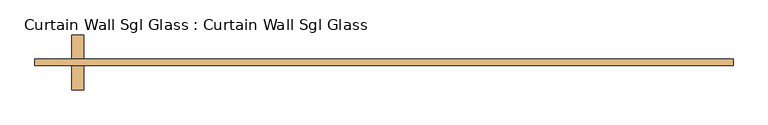
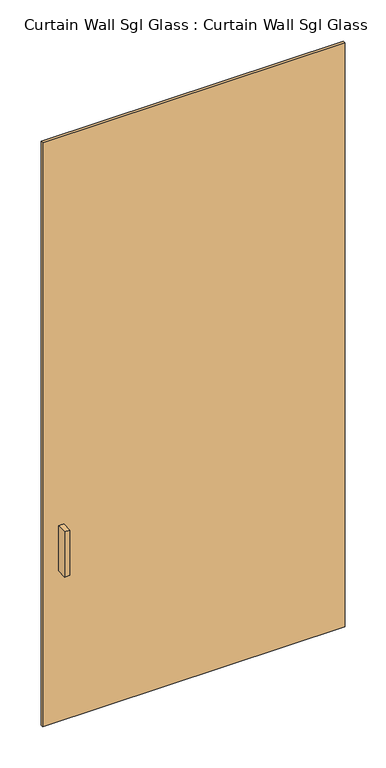
"""IFC4 building model written with IfcOpenShell, lengths in millimetres: door geometry, Curtain Wall Sgl Glass : Curtain Wall Sgl Glass."""

from ifc_helpers import new_model, si_unit, frame, origin, origin_with_axes, place, context, project, spatial, polyline, outline, extrude, source, transform, mapped, element, save


def curtain_wall_sgl_glass_curtain_wall_sgl_glass_b8118105(model_context):
    return source(origin(), model_context, "Body", "SweptSolid", [
        extrude(outline(polyline([(-621.6871469, 12.7), (-621.6871469, -38.1), (-647.0871469, -38.1), (-647.0871469, 12.7), (-621.6871469, 12.7)])), frame((0.0, 0.0, 762.0), z_axis=(0.0, 0.0, 1.0), x_axis=(1.0, 0.0, 0.0)), (0.0, 0.0, 1.0), 228.6),
        extrude(outline(polyline([(-647.0871469, -101.6), (-647.0871469, -50.8), (-621.6871469, -50.8), (-621.6871469, -101.6), (-647.0871469, -101.6)])), frame((0.0, 0.0, 762.0), z_axis=(0.0, 0.0, 1.0), x_axis=(1.0, 0.0, 0.0)), (0.0, 0.0, 1.0), 228.6),
        extrude(outline(polyline([(723.2871469, -50.8), (-723.2871469, -50.8), (-723.2871469, -38.1), (723.2871469, -38.1), (723.2871469, -50.8)])), origin_with_axes(), (0.0, 0.0, 1.0), 2952.75),
    ])


if __name__ == "__main__":
    model = new_model("IFC4")
    model_context = context("Model", 3, world=origin())
    ifc_project = project(units=[si_unit("LENGTHUNIT", "METRE", prefix="MILLI")], contexts=[model_context])
    site = spatial("IfcSite", under=ifc_project)
    building = spatial("IfcBuilding", under=site)
    placement = place(None, origin())
    curtain_wall_sgl_glass_curtain_wall_sgl_glass_shape = curtain_wall_sgl_glass_curtain_wall_sgl_glass_b8118105(model_context)
    element("IfcDoor", 1, ObjectType="Curtain Wall Sgl Glass : Curtain Wall Sgl Glass", at=placement, inside=building, context=model_context, shape_type="MappedRepresentation", body=[
        mapped(curtain_wall_sgl_glass_curtain_wall_sgl_glass_shape, transform((0.0, 0.0, 0.0), x_axis=(1.0, 0.0, 0.0), y_axis=(0.0, 1.0, 0.0), z_axis=(0.0, 0.0, 1.0))),
    ])
    save(model, "model.ifc")

# Revit data of these elements
# Type "Curtain Wall Sgl Glass : Curtain Wall Sgl Glass"
#   Type Mark = "8"
#   Assembly Code = "B2030100"
#   Offset = 0' - 2"
#   Function = 1
#   Handle Material = Metal - Aluminum
#   Glazing Material = Glass
# Element 1 (IfcDoor, "Curtain Wall Sgl Glass : Curtain Wall Sgl Glass")
#   Materials on its faces: "Metal - Aluminum", "Glass"
# Materials
#   "Metal - Aluminum": class "Metal", colour RGB 247 247 247, transparency 0
#   "Glass": class "Unassigned", colour RGB 147 173 200, transparency 0.7, Cost = 0
